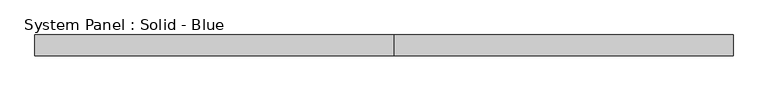
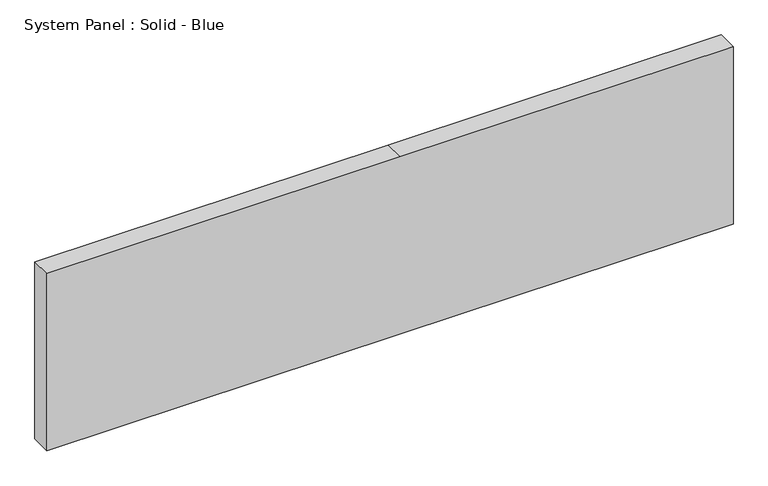
"""IFC4 building model written with IfcOpenShell, lengths in millimetres: plate geometry, System Panel : Solid - Blue."""

import ifcopenshell
import ifcopenshell.guid

model = None  # the IFC model being written
_history = None  # IfcOwnerHistory: only IFC2X3 demands one
_inside = {}  # id of a spatial element -> (the spatial element, [elements in it])
_under = {}  # id of a project, library or spatial element -> (it, [spatial elements below it])
_declared = {}  # id of a project -> (the project, [libraries it declares])
_typed = {}  # id of a type object -> (the type object, [elements of that type])
_made_of = {}  # id of a material, layer set ... -> (it, [elements and type objects made of it])


def new_model(schema):
    """Start an empty IFC model of exactly this schema.

    Asked for "IFC4X3", IfcOpenShell would pick the latest addendum, in which some entities
    have other attributes; the version numbers below select the first issue.
    IFC2X3 requires an IfcOwnerHistory on every rooted entity: one is made here for all.
    """
    global model, _history
    if schema == "IFC4X3":
        model = ifcopenshell.file(schema_version=(4, 3, 0, 0))
    else:
        model = ifcopenshell.file(schema=schema)
    _inside.clear()
    _under.clear()
    _declared.clear()
    _typed.clear()
    _made_of.clear()
    _history = None
    if model.schema == "IFC2X3":
        org = make("IfcOrganization", Name="unknown")
        user = make(
            "IfcPersonAndOrganization",
            ThePerson=make("IfcPerson", FamilyName="unknown"),
            TheOrganization=org,
        )
        app = make(
            "IfcApplication",
            ApplicationDeveloper=org,
            Version="unknown",
            ApplicationFullName="unknown",
            ApplicationIdentifier="unknown",
        )
        _history = make(
            "IfcOwnerHistory",
            OwningUser=user,
            OwningApplication=app,
            ChangeAction="ADDED",
            CreationDate=0,
        )
    return model


def make(cls, **values):
    """One entity of the class cls with the attributes given. An attribute that is None is left unset."""
    return model.create_entity(
        cls, **{name: value for name, value in values.items() if value is not None}
    )


def rooted(cls, **values):
    """An entity with a GlobalId (a new one), such as an element, a storey or a relation."""
    return make(cls, GlobalId=ifcopenshell.guid.new(), OwnerHistory=_history, **values)


def si_unit(unit_type, name, prefix=None):
    """IfcSIUnit, for example si_unit("LENGTHUNIT", "METRE", prefix="MILLI")."""
    return make("IfcSIUnit", UnitType=unit_type, Prefix=prefix, Name=name)


def assignment(units):
    """IfcUnitAssignment: the units of a project."""
    return None if units is None else make("IfcUnitAssignment", Units=units)


def point(xyz):
    """IfcCartesianPoint."""
    return None if xyz is None else make("IfcCartesianPoint", Coordinates=xyz)


def direction(xyz):
    """IfcDirection."""
    return None if xyz is None else make("IfcDirection", DirectionRatios=xyz)


def frame(location, z_axis=None, x_axis=None):
    """IfcAxis2Placement3D, a coordinate frame: its origin and axes. An axis left out is left unset."""
    return make(
        "IfcAxis2Placement3D",
        Location=point(location),
        Axis=direction(z_axis),
        RefDirection=direction(x_axis),
    )


def origin():
    """The frame at (0, 0, 0) with its axes left unset."""
    return frame((0.0, 0.0, 0.0))


def place(relative_to, where):
    """IfcLocalPlacement: puts the frame where relative to a parent placement (None: the world)."""
    return make(
        "IfcLocalPlacement", PlacementRelTo=relative_to, RelativePlacement=where
    )


def context(
    kind, dimensions, precision=None, world=None, true_north=None, identifier=None
):
    """IfcGeometricRepresentationContext, for example the 3D "Model" context."""
    return make(
        "IfcGeometricRepresentationContext",
        ContextIdentifier=identifier,
        ContextType=kind,
        CoordinateSpaceDimension=dimensions,
        Precision=precision,
        WorldCoordinateSystem=world,
        TrueNorth=true_north,
    )


def project(units=None, contexts=None):
    """IfcProject with its units and contexts."""
    return rooted(
        "IfcProject",
        Name="project",
        RepresentationContexts=contexts,
        UnitsInContext=assignment(units),
    )


def spatial(cls, under=None, at=None, **own):
    """A site, building, storey or space (cls), placed at a placement, below another one or the project."""
    s = rooted(cls, ObjectPlacement=at, **own)
    if under is not None:
        _under.setdefault(under.id(), (under, []))[1].append(s)
    return s


def polyline(points):
    """IfcPolyline through the points."""
    return make("IfcPolyline", Points=[point(p) for p in points])


def outline(outer, holes=None, kind="AREA"):
    """IfcArbitraryClosedProfileDef: a profile drawn as a closed curve; with holes, ...WithVoids."""
    if holes is None:
        return make("IfcArbitraryClosedProfileDef", ProfileType=kind, OuterCurve=outer)
    return make(
        "IfcArbitraryProfileDefWithVoids",
        ProfileType=kind,
        OuterCurve=outer,
        InnerCurves=holes,
    )


def extrude(swept, where, along, depth):
    """IfcExtrudedAreaSolid: the profile swept, set in the frame where, extruded along a direction by depth."""
    return make(
        "IfcExtrudedAreaSolid",
        SweptArea=swept,
        Position=where,
        ExtrudedDirection=direction(along),
        Depth=depth,
    )


def shape(context_of_items, identifier, shape_type, items):
    """IfcShapeRepresentation: the items that make up one representation, for example the "Body"."""
    return make(
        "IfcShapeRepresentation",
        ContextOfItems=context_of_items,
        RepresentationIdentifier=identifier,
        RepresentationType=shape_type,
        Items=items,
    )


def source(mapping_origin, context_of_items, identifier, shape_type, items):
    """IfcRepresentationMap: a shape defined once, which mapped items show again and again."""
    return make(
        "IfcRepresentationMap",
        MappingOrigin=mapping_origin,
        MappedRepresentation=shape(context_of_items, identifier, shape_type, items),
    )


def transform(
    local_origin,
    x_axis=None,
    y_axis=None,
    z_axis=None,
    scale=None,
    scale2=None,
    scale3=None,
    uniform=True,
):
    """IfcCartesianTransformationOperator3D, or its non-uniform kind. x_axis, y_axis, z_axis: its Axis1, 2, 3."""
    if uniform:
        return make(
            "IfcCartesianTransformationOperator3D",
            Axis1=direction(x_axis),
            Axis2=direction(y_axis),
            LocalOrigin=point(local_origin),
            Scale=scale,
            Axis3=direction(z_axis),
        )
    return make(
        "IfcCartesianTransformationOperator3DnonUniform",
        Axis1=direction(x_axis),
        Axis2=direction(y_axis),
        LocalOrigin=point(local_origin),
        Scale=scale,
        Axis3=direction(z_axis),
        Scale2=scale2,
        Scale3=scale3,
    )


def mapped(mapping_source, mapping_target):
    """IfcMappedItem: shows the shape of a source again, moved by a transform."""
    return make(
        "IfcMappedItem", MappingSource=mapping_source, MappingTarget=mapping_target
    )


def made_of(thing, what):
    """Note that an element or type object is made of a material, layer set ...; save() writes the relation."""
    if what is not None:
        _made_of.setdefault(what.id(), (what, []))[1].append(thing)
    return thing


def element(
    cls,
    number,
    at=None,
    inside=None,
    cuts=None,
    type_object=None,
    material=None,
    context=None,
    identifier="Body",
    shape_type=None,
    held_by="IfcProductDefinitionShape",
    body=None,
    shapes=None,
    **own,
):
    """One element of the class cls, such as IfcWall. Its Tag is "e" and its number.

    at: its placement. inside: the storey or other place that contains it. cuts: it is an
    opening in that element (IfcRelVoidsElement). A single representation is given by context,
    identifier, shape_type and body (its items); several are given by shapes. held_by: the class
    of the entity that holds the representations. save() writes the other relations.
    """
    e = rooted(cls, Tag="e%d" % number, ObjectPlacement=at, **own)
    if body is not None:
        shapes = [shape(context, identifier, shape_type, body)]
    if shapes is not None:
        e.Representation = make(held_by, Representations=shapes)
    if inside is not None:
        _inside.setdefault(inside.id(), (inside, []))[1].append(e)
    if cuts is not None:
        rooted(
            "IfcRelVoidsElement", RelatingBuildingElement=cuts, RelatedOpeningElement=e
        )
    if type_object is not None:
        _typed.setdefault(type_object.id(), (type_object, []))[1].append(e)
    return made_of(e, material)


def aggregate(whole, parts):
    """IfcRelAggregates: a whole, such as a stair, and the parts it consists of."""
    return rooted("IfcRelAggregates", RelatingObject=whole, RelatedObjects=parts)


def save(model, path):
    """Write the relations noted so far, then the file.

    IfcRelAggregates (storeys below a building ...), IfcRelContainedInSpatialStructure (elements
    in a storey), IfcRelDefinesByType, IfcRelAssociatesMaterial and IfcRelDeclares: one each for
    every whole, place, type object, material and project.
    """
    for whole, parts in _under.values():
        aggregate(whole, parts)
    for where, things in _inside.values():
        rooted(
            "IfcRelContainedInSpatialStructure",
            RelatedElements=things,
            RelatingStructure=where,
        )
    for kind, things in _typed.values():
        rooted("IfcRelDefinesByType", RelatedObjects=things, RelatingType=kind)
    for what, things in _made_of.values():
        rooted("IfcRelAssociatesMaterial", RelatedObjects=things, RelatingMaterial=what)
    for by, libraries in _declared.values():
        rooted("IfcRelDeclares", RelatingContext=by, RelatedDefinitions=libraries)
    model.write(path)


def system_panel_solid_blue_23037680(model_context):
    return source(origin(), model_context, "Body", "SweptSolid", [
        extrude(outline(polyline([(0.0, -1057.7285714), (0.0, 31.75), (0.0, 1057.7285714), (577.85, 1057.7285714), (577.85, 31.75), (577.85, -1057.7285714), (0.0, -1057.7285714)])), frame((0.0, -19.05, 0.0), z_axis=(0.0, 1.0, 0.0), x_axis=(0.0, 0.0, 1.0)), (0.0, 0.0, 1.0), 63.5),
    ])


if __name__ == "__main__":
    model = new_model("IFC4")
    model_context = context("Model", 3, world=origin())
    ifc_project = project(units=[si_unit("LENGTHUNIT", "METRE", prefix="MILLI")], contexts=[model_context])
    site = spatial("IfcSite", under=ifc_project)
    building = spatial("IfcBuilding", under=site)
    placement = place(None, origin())
    system_panel_solid_blue_shape = system_panel_solid_blue_23037680(model_context)
    element("IfcPlate", 1, ObjectType="System Panel : Solid - Blue", at=placement, inside=building, context=model_context, shape_type="MappedRepresentation", body=[
        mapped(system_panel_solid_blue_shape, transform((0.0, 0.0, 0.0), x_axis=(1.0, 0.0, 0.0), y_axis=(0.0, 1.0, 0.0), z_axis=(0.0, 0.0, 1.0))),
    ])
    save(model, "model.ifc")

# Revit data of these elements
# Project information
#   SR Document GUID = "4c5931b3-dab8-40a9-800d-cf79e49c7e77"
# Element 1 (IfcPlate, "System Panel : Solid - Blue")
#   Materials on its faces: "Blue Panel"
# Materials
#   "Blue Panel": class "Unassigned", colour RGB 0 0 160, transparency 0
